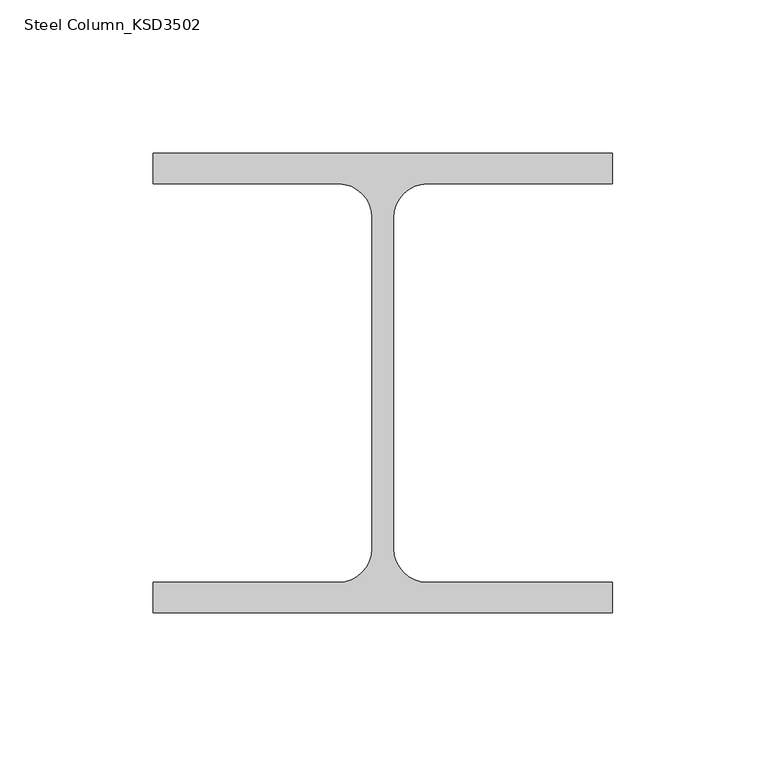
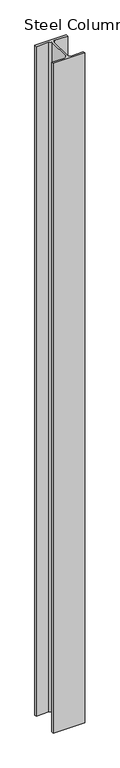
"""IFC4 building model written with IfcOpenShell, lengths in millimetres: column geometry, Steel Column_KSD3502 : H_SC_ASC_H-150×150x7x10."""

from ifc_helpers import new_model, si_unit, point, frame, frame_2d, origin, place, context, project, spatial, polyline, circle_curve, trimmed, segment, composite_curve, outline, extrude, source, transform, mapped, element, save


def steel_column_ksd3502_781554eb(model_context):
    return source(origin(), model_context, "Body", "SweptSolid", [
        extrude(outline(composite_curve([segment(polyline([(75.0, 75.0), (75.0, 65.0), (14.5, 65.0)]), True, "CONTINUOUS"), segment(trimmed(circle_curve(frame_2d((14.5, 54.0)), 11.0), [point((14.5, 65.0))], [point((3.5, 54.0))], True, "CARTESIAN"), True, "CONTINUOUS"), segment(polyline([(3.5, 54.0), (3.5, -54.0)]), True, "CONTINUOUS"), segment(trimmed(circle_curve(frame_2d((14.5, -54.0)), 11.0), [point((3.5, -54.0))], [point((14.5, -65.0))], True, "CARTESIAN"), True, "CONTINUOUS"), segment(polyline([(14.5, -65.0), (75.0, -65.0), (75.0, -75.0), (-75.0, -75.0), (-75.0, -65.0), (-14.5, -65.0)]), True, "CONTINUOUS"), segment(trimmed(circle_curve(frame_2d((-14.5, -54.0)), 11.0), [point((-14.5, -65.0))], [point((-3.5, -54.0))], True, "CARTESIAN"), True, "CONTINUOUS"), segment(polyline([(-3.5, -54.0), (-3.5, 54.0)]), True, "CONTINUOUS"), segment(trimmed(circle_curve(frame_2d((-14.5, 54.0)), 11.0), [point((-3.5, 54.0))], [point((-14.5, 65.0))], True, "CARTESIAN"), True, "CONTINUOUS"), segment(polyline([(-14.5, 65.0), (-75.0, 65.0), (-75.0, 75.0), (75.0, 75.0)]), True, "CONTINUOUS")], self_intersect=False)), frame((0.0, 0.0, 599.9720055), z_axis=(0.0, 0.0, 1.0), x_axis=(1.0, 0.0, 0.0)), (0.0, 0.0, 1.0), 3368.0),
    ])


if __name__ == "__main__":
    model = new_model("IFC4")
    model_context = context("Model", 3, world=origin())
    ifc_project = project(units=[si_unit("LENGTHUNIT", "METRE", prefix="MILLI")], contexts=[model_context])
    site = spatial("IfcSite", under=ifc_project)
    building = spatial("IfcBuilding", under=site)
    placement = place(None, origin())
    steel_column_ksd3502_shape = steel_column_ksd3502_781554eb(model_context)
    element("IfcColumn", 1, ObjectType="Steel Column_KSD3502 : H_SC_ASC_H-150×150x7x10", at=placement, inside=building, context=model_context, shape_type="MappedRepresentation", body=[
        mapped(steel_column_ksd3502_shape, transform((0.0, 0.0, 0.0), x_axis=(1.0, 0.0, 0.0), y_axis=(0.0, 1.0, 0.0), z_axis=(0.0, 0.0, 1.0))),
    ])
    save(model, "model.ifc")

# Revit data of these elements
# Type "Steel Column_KSD3502 : H_SC_ASC_H-150×150x7x10"
#   Width = 15.0 cm
#   Web Thickness = 0.7 cm
#   Web Fillet = 1.1 cm
#   Warping Constant = 27562.5 cm⁶
#   Torsional Moment of Inertia = 11.6007 cm⁴
#   Section Area = 40.14 cm²
#   Plastic Modulus weak axis = 115.0 cm³
#   Plastic Modulus strong axis = 246.0 cm³
#   Perimeter = 1.27 m²/m
#   Nominal Weight = 31.50 kgf/m
#   Moment of Inertia weak axis = 563.00 cm⁴
#   Moment of Inertia strong axis = 1640.00 cm⁴
#   Height = 15.0 cm
#   Flange Thickness = 1.0 cm
#   Elastic Modulus weak axis = 75.1 cm³
#   Elastic Modulus strong axis = 219.0 cm³
#   Centroid Vertical = 7.5 cm
#   Centroid Horizontal = 7.5 cm
#   Bolt Spacing = 13.97 cm
#   Structural Material [instance default] = Steel, 45-345
#   Section Name Key = ""
#   Assembly Code = ""
# Element 1 (IfcColumn, "Steel Column_KSD3502 : H_SC_ASC_H-150×150x7x10")
#   Structural Material = A03AD029-00005_Anchor Bolt (Installation only)_M24
#   Materials on its faces: "A03AD029-00005_Anchor Bolt (Installation only)_M24"
# Materials
#   "Steel, 45-345": class "Metal", colour RGB 189 187 185, transparency 0, Description = "Steel 345 MPa", Cost = 0
#   "A03AD029-00005_Anchor Bolt (Installation only)_M24": class "Unassigned", colour RGB 84 83 81, transparency 0, Cost = 0
